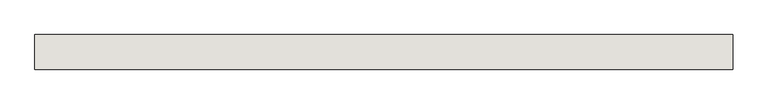
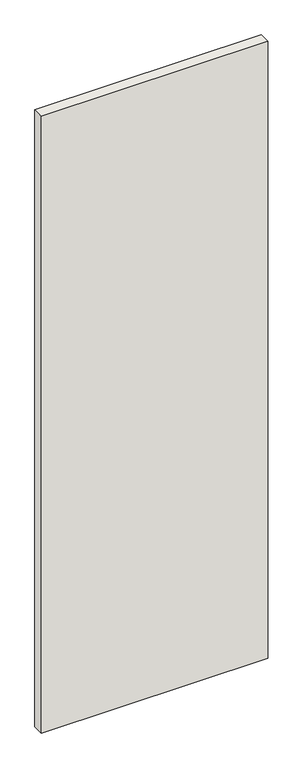
"""IFC4 building model written with IfcOpenShell, lengths in millimetres: wall geometry, 0_3d."""

from ifc_helpers import new_model, si_unit, origin, origin_with_axes, place, context, project, spatial, polyline, outline, extrude, source, transform, mapped, element, save


def wall_e279f2a4(model_context):
    return source(origin(), model_context, "Body", "SweptSolid", [
        extrude(outline(polyline([(1000.0, 50.0), (1000.0, 0.0), (0.0, 0.0), (0.0, 50.0), (1000.0, 50.0)])), origin_with_axes(), (0.0, 0.0, 1.0), 2880.0),
    ])


if __name__ == "__main__":
    model = new_model("IFC4")
    model_context = context("Model", 3, world=origin())
    ifc_project = project(units=[si_unit("LENGTHUNIT", "METRE", prefix="MILLI")], contexts=[model_context])
    site = spatial("IfcSite", under=ifc_project)
    building = spatial("IfcBuilding", under=site)
    placement = place(None, origin())
    wall_shape = wall_e279f2a4(model_context)
    element("IfcWall", 1, ObjectType="0_3d", at=placement, inside=building, context=model_context, shape_type="MappedRepresentation", body=[
        mapped(wall_shape, transform((0.0, 0.0, 0.0), x_axis=(1.0, 0.0, 0.0), y_axis=(0.0, 1.0, 0.0), z_axis=(0.0, 0.0, 1.0))),
    ])
    save(model, "model.ifc")

# Revit data of these elements
# Element 1 (IfcWall, "0_3d")
#   Materials on its faces: "glas"
# Materials
#   "glas": class "Unassigned", colour RGB 250 253 254, transparency 0.95
